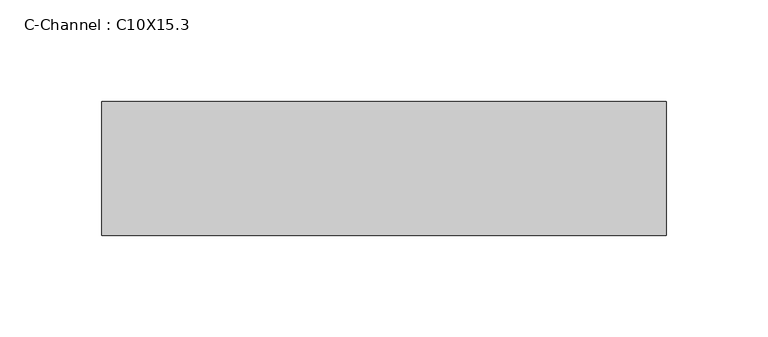
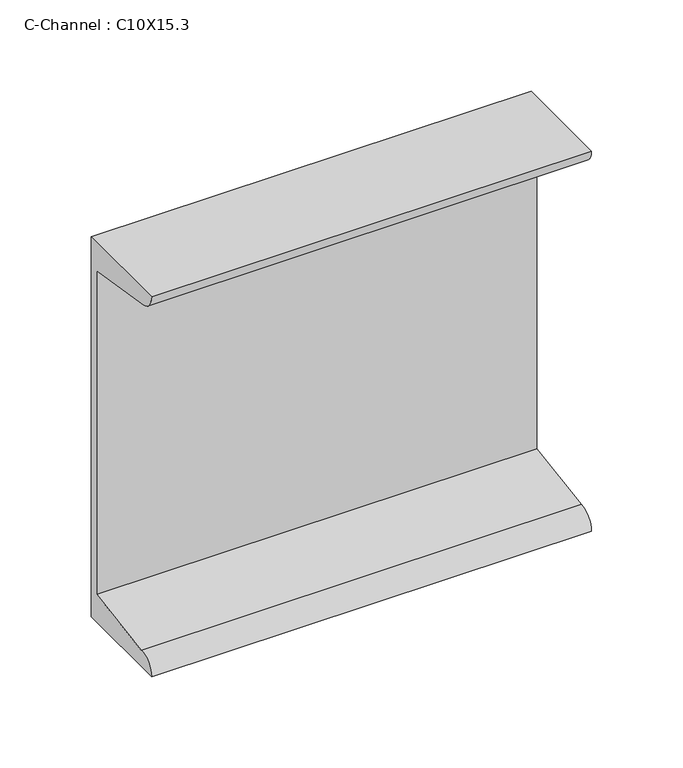
"""IFC4 building model written with IfcOpenShell, lengths in millimetres: beam geometry, C-Channel : C10X15.3."""

import ifcopenshell
import ifcopenshell.guid

model = None  # the IFC model being written
_history = None  # IfcOwnerHistory: only IFC2X3 demands one
_inside = {}  # id of a spatial element -> (the spatial element, [elements in it])
_under = {}  # id of a project, library or spatial element -> (it, [spatial elements below it])
_declared = {}  # id of a project -> (the project, [libraries it declares])
_typed = {}  # id of a type object -> (the type object, [elements of that type])
_made_of = {}  # id of a material, layer set ... -> (it, [elements and type objects made of it])


def new_model(schema):
    """Start an empty IFC model of exactly this schema.

    Asked for "IFC4X3", IfcOpenShell would pick the latest addendum, in which some entities
    have other attributes; the version numbers below select the first issue.
    IFC2X3 requires an IfcOwnerHistory on every rooted entity: one is made here for all.
    """
    global model, _history
    if schema == "IFC4X3":
        model = ifcopenshell.file(schema_version=(4, 3, 0, 0))
    else:
        model = ifcopenshell.file(schema=schema)
    _inside.clear()
    _under.clear()
    _declared.clear()
    _typed.clear()
    _made_of.clear()
    _history = None
    if model.schema == "IFC2X3":
        org = make("IfcOrganization", Name="unknown")
        user = make(
            "IfcPersonAndOrganization",
            ThePerson=make("IfcPerson", FamilyName="unknown"),
            TheOrganization=org,
        )
        app = make(
            "IfcApplication",
            ApplicationDeveloper=org,
            Version="unknown",
            ApplicationFullName="unknown",
            ApplicationIdentifier="unknown",
        )
        _history = make(
            "IfcOwnerHistory",
            OwningUser=user,
            OwningApplication=app,
            ChangeAction="ADDED",
            CreationDate=0,
        )
    return model


def make(cls, **values):
    """One entity of the class cls with the attributes given. An attribute that is None is left unset."""
    return model.create_entity(
        cls, **{name: value for name, value in values.items() if value is not None}
    )


def rooted(cls, **values):
    """An entity with a GlobalId (a new one), such as an element, a storey or a relation."""
    return make(cls, GlobalId=ifcopenshell.guid.new(), OwnerHistory=_history, **values)


def si_unit(unit_type, name, prefix=None):
    """IfcSIUnit, for example si_unit("LENGTHUNIT", "METRE", prefix="MILLI")."""
    return make("IfcSIUnit", UnitType=unit_type, Prefix=prefix, Name=name)


def assignment(units):
    """IfcUnitAssignment: the units of a project."""
    return None if units is None else make("IfcUnitAssignment", Units=units)


def point(xyz):
    """IfcCartesianPoint."""
    return None if xyz is None else make("IfcCartesianPoint", Coordinates=xyz)


def direction(xyz):
    """IfcDirection."""
    return None if xyz is None else make("IfcDirection", DirectionRatios=xyz)


def frame(location, z_axis=None, x_axis=None):
    """IfcAxis2Placement3D, a coordinate frame: its origin and axes. An axis left out is left unset."""
    return make(
        "IfcAxis2Placement3D",
        Location=point(location),
        Axis=direction(z_axis),
        RefDirection=direction(x_axis),
    )


def frame_2d(location, x_axis=None):
    """IfcAxis2Placement2D, a coordinate frame in the plane: its origin and x axis."""
    return make(
        "IfcAxis2Placement2D", Location=point(location), RefDirection=direction(x_axis)
    )


def origin():
    """The frame at (0, 0, 0) with its axes left unset."""
    return frame((0.0, 0.0, 0.0))


def place(relative_to, where):
    """IfcLocalPlacement: puts the frame where relative to a parent placement (None: the world)."""
    return make(
        "IfcLocalPlacement", PlacementRelTo=relative_to, RelativePlacement=where
    )


def context(
    kind, dimensions, precision=None, world=None, true_north=None, identifier=None
):
    """IfcGeometricRepresentationContext, for example the 3D "Model" context."""
    return make(
        "IfcGeometricRepresentationContext",
        ContextIdentifier=identifier,
        ContextType=kind,
        CoordinateSpaceDimension=dimensions,
        Precision=precision,
        WorldCoordinateSystem=world,
        TrueNorth=true_north,
    )


def project(units=None, contexts=None):
    """IfcProject with its units and contexts."""
    return rooted(
        "IfcProject",
        Name="project",
        RepresentationContexts=contexts,
        UnitsInContext=assignment(units),
    )


def spatial(cls, under=None, at=None, **own):
    """A site, building, storey or space (cls), placed at a placement, below another one or the project."""
    s = rooted(cls, ObjectPlacement=at, **own)
    if under is not None:
        _under.setdefault(under.id(), (under, []))[1].append(s)
    return s


def polyline(points):
    """IfcPolyline through the points."""
    return make("IfcPolyline", Points=[point(p) for p in points])


def circle_curve(where, radius):
    """IfcCircle in the frame where."""
    return make("IfcCircle", Position=where, Radius=radius)


def trimmed(basis, trim1, trim2, sense, master):
    """IfcTrimmedCurve: the piece of a basis curve between two trims."""
    return make(
        "IfcTrimmedCurve",
        BasisCurve=basis,
        Trim1=trim1,
        Trim2=trim2,
        SenseAgreement=sense,
        MasterRepresentation=master,
    )


def segment(curve, same_sense, transition):
    """IfcCompositeCurveSegment."""
    return make(
        "IfcCompositeCurveSegment",
        Transition=transition,
        SameSense=same_sense,
        ParentCurve=curve,
    )


def composite_curve(segments, self_intersect=None):
    """IfcCompositeCurve: segments joined end to end."""
    return make("IfcCompositeCurve", Segments=segments, SelfIntersect=self_intersect)


def outline(outer, holes=None, kind="AREA"):
    """IfcArbitraryClosedProfileDef: a profile drawn as a closed curve; with holes, ...WithVoids."""
    if holes is None:
        return make("IfcArbitraryClosedProfileDef", ProfileType=kind, OuterCurve=outer)
    return make(
        "IfcArbitraryProfileDefWithVoids",
        ProfileType=kind,
        OuterCurve=outer,
        InnerCurves=holes,
    )


def extrude(swept, where, along, depth):
    """IfcExtrudedAreaSolid: the profile swept, set in the frame where, extruded along a direction by depth."""
    return make(
        "IfcExtrudedAreaSolid",
        SweptArea=swept,
        Position=where,
        ExtrudedDirection=direction(along),
        Depth=depth,
    )


def shape(context_of_items, identifier, shape_type, items):
    """IfcShapeRepresentation: the items that make up one representation, for example the "Body"."""
    return make(
        "IfcShapeRepresentation",
        ContextOfItems=context_of_items,
        RepresentationIdentifier=identifier,
        RepresentationType=shape_type,
        Items=items,
    )


def source(mapping_origin, context_of_items, identifier, shape_type, items):
    """IfcRepresentationMap: a shape defined once, which mapped items show again and again."""
    return make(
        "IfcRepresentationMap",
        MappingOrigin=mapping_origin,
        MappedRepresentation=shape(context_of_items, identifier, shape_type, items),
    )


def transform(
    local_origin,
    x_axis=None,
    y_axis=None,
    z_axis=None,
    scale=None,
    scale2=None,
    scale3=None,
    uniform=True,
):
    """IfcCartesianTransformationOperator3D, or its non-uniform kind. x_axis, y_axis, z_axis: its Axis1, 2, 3."""
    if uniform:
        return make(
            "IfcCartesianTransformationOperator3D",
            Axis1=direction(x_axis),
            Axis2=direction(y_axis),
            LocalOrigin=point(local_origin),
            Scale=scale,
            Axis3=direction(z_axis),
        )
    return make(
        "IfcCartesianTransformationOperator3DnonUniform",
        Axis1=direction(x_axis),
        Axis2=direction(y_axis),
        LocalOrigin=point(local_origin),
        Scale=scale,
        Axis3=direction(z_axis),
        Scale2=scale2,
        Scale3=scale3,
    )


def mapped(mapping_source, mapping_target):
    """IfcMappedItem: shows the shape of a source again, moved by a transform."""
    return make(
        "IfcMappedItem", MappingSource=mapping_source, MappingTarget=mapping_target
    )


def made_of(thing, what):
    """Note that an element or type object is made of a material, layer set ...; save() writes the relation."""
    if what is not None:
        _made_of.setdefault(what.id(), (what, []))[1].append(thing)
    return thing


def element(
    cls,
    number,
    at=None,
    inside=None,
    cuts=None,
    type_object=None,
    material=None,
    context=None,
    identifier="Body",
    shape_type=None,
    held_by="IfcProductDefinitionShape",
    body=None,
    shapes=None,
    **own,
):
    """One element of the class cls, such as IfcWall. Its Tag is "e" and its number.

    at: its placement. inside: the storey or other place that contains it. cuts: it is an
    opening in that element (IfcRelVoidsElement). A single representation is given by context,
    identifier, shape_type and body (its items); several are given by shapes. held_by: the class
    of the entity that holds the representations. save() writes the other relations.
    """
    e = rooted(cls, Tag="e%d" % number, ObjectPlacement=at, **own)
    if body is not None:
        shapes = [shape(context, identifier, shape_type, body)]
    if shapes is not None:
        e.Representation = make(held_by, Representations=shapes)
    if inside is not None:
        _inside.setdefault(inside.id(), (inside, []))[1].append(e)
    if cuts is not None:
        rooted(
            "IfcRelVoidsElement", RelatingBuildingElement=cuts, RelatedOpeningElement=e
        )
    if type_object is not None:
        _typed.setdefault(type_object.id(), (type_object, []))[1].append(e)
    return made_of(e, material)


def aggregate(whole, parts):
    """IfcRelAggregates: a whole, such as a stair, and the parts it consists of."""
    return rooted("IfcRelAggregates", RelatingObject=whole, RelatedObjects=parts)


def save(model, path):
    """Write the relations noted so far, then the file.

    IfcRelAggregates (storeys below a building ...), IfcRelContainedInSpatialStructure (elements
    in a storey), IfcRelDefinesByType, IfcRelAssociatesMaterial and IfcRelDeclares: one each for
    every whole, place, type object, material and project.
    """
    for whole, parts in _under.values():
        aggregate(whole, parts)
    for where, things in _inside.values():
        rooted(
            "IfcRelContainedInSpatialStructure",
            RelatedElements=things,
            RelatingStructure=where,
        )
    for kind, things in _typed.values():
        rooted("IfcRelDefinesByType", RelatedObjects=things, RelatingType=kind)
    for what, things in _made_of.values():
        rooted("IfcRelAssociatesMaterial", RelatedObjects=things, RelatingMaterial=what)
    for by, libraries in _declared.values():
        rooted("IfcRelDeclares", RelatingContext=by, RelatedDefinitions=libraries)
    model.write(path)


def c_channel_c10x15_3_72e663a1(model_context):
    return source(origin(), model_context, "Body", "SweptSolid", [
        extrude(outline(composite_curve([segment(polyline([(16.1036, 127.0), (16.1036, -127.0), (-49.9364, -127.0)]), True, "CONTINUOUS"), segment(trimmed(circle_curve(frame_2d((-38.862, -127.0)), 11.0744), [point((-49.9364, -127.0))], [point((-38.862, -115.9256))], False, "CARTESIAN"), True, "CONTINUOUS"), segment(polyline([(-38.862, -115.9256), (10.0076, -108.1854158), (10.0076, 108.1854158), (-38.862, 115.9256)]), True, "CONTINUOUS"), segment(trimmed(circle_curve(frame_2d((-38.862, 127.0)), 11.0744), [point((-38.862, 115.9256))], [point((-49.9364, 127.0))], False, "CARTESIAN"), True, "CONTINUOUS"), segment(polyline([(-49.9364, 127.0), (16.1036, 127.0)]), True, "CONTINUOUS")], self_intersect=False)), frame((-125.73, 0.0, 0.0), z_axis=(1.0, 0.0, 0.0), x_axis=(0.0, 1.0, 0.0)), (0.0, 0.0, 1.0), 278.13),
    ])


if __name__ == "__main__":
    model = new_model("IFC4")
    model_context = context("Model", 3, world=origin())
    ifc_project = project(units=[si_unit("LENGTHUNIT", "METRE", prefix="MILLI")], contexts=[model_context])
    site = spatial("IfcSite", under=ifc_project)
    building = spatial("IfcBuilding", under=site)
    placement = place(None, origin())
    c_channel_c10x15_3_shape = c_channel_c10x15_3_72e663a1(model_context)
    element("IfcBeam", 1, ObjectType="C-Channel : C10X15.3", at=placement, inside=building, context=model_context, shape_type="MappedRepresentation", body=[
        mapped(c_channel_c10x15_3_shape, transform((0.0, 0.0, 0.0), x_axis=(1.0, 0.0, 0.0), y_axis=(0.0, 1.0, 0.0), z_axis=(0.0, 0.0, 1.0))),
    ])
    save(model, "model.ifc")

# Revit data of these elements
# Type "C-Channel : C10X15.3"
#   Assembly Code = "B10"
#   W = 15.3
#   Length [instance default] = 5' - 0"
#   bf = 0' - 2.6"
#   d = 0' - 10"
#   tf = 0' - 0.436"
#   tw = 0' - 0.24"
#   x = 0' - 0.634"
#   A = 0.0311111 SF
#   Structural Material [instance default] = Steel ASTM A36
# Element 1 (IfcBeam, "C-Channel : C10X15.3")
#   Structural Material = Steel ASTM A992
#   Materials on its faces: "Steel ASTM A992"
# Materials
#   "Steel ASTM A36": class "Metal", colour RGB 199 199 199, transparency 0, Description = "Structural steel, ASTM A36 Grade B, mill finish", Cost = 0
#   "Steel ASTM A992": class "Metal", colour RGB 199 199 199, transparency 0, Description = "Structural steel 50ksi", Cost = 0
